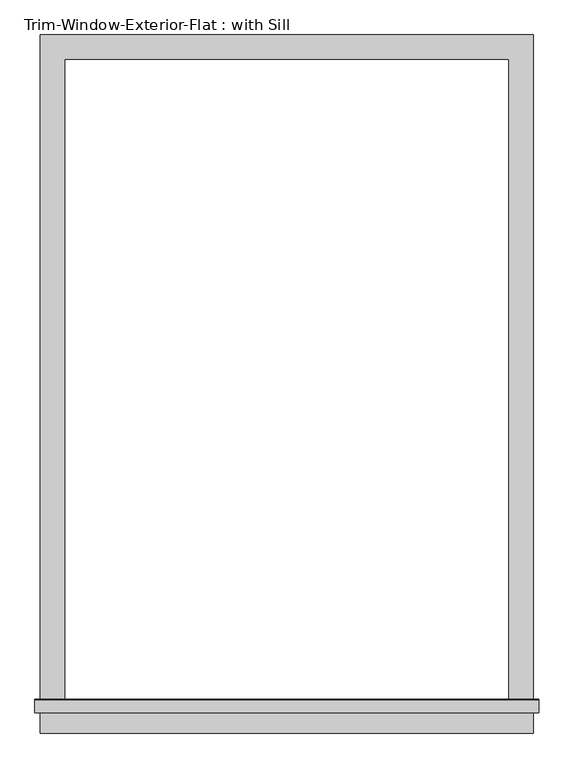
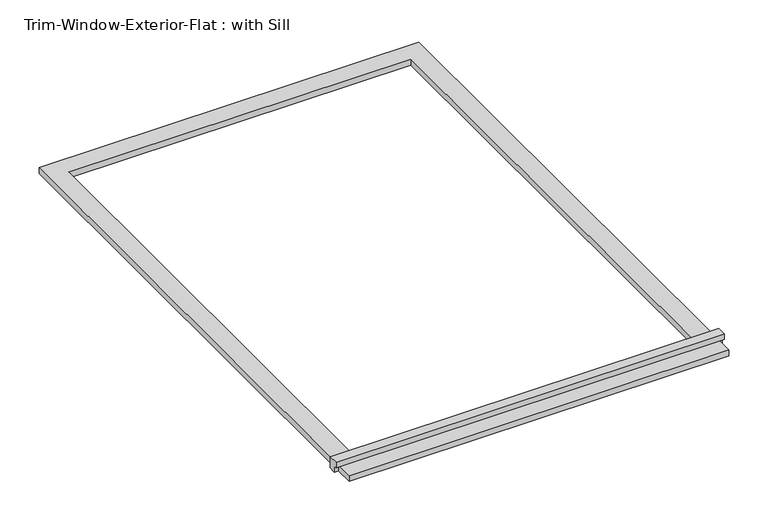
"""IFC4 building model written with IfcOpenShell, lengths in millimetres: proxy geometry, Trim-Window-Exterior-Flat : with Sill."""

import ifcopenshell
import ifcopenshell.guid

model = None  # the IFC model being written
_history = None  # IfcOwnerHistory: only IFC2X3 demands one
_inside = {}  # id of a spatial element -> (the spatial element, [elements in it])
_under = {}  # id of a project, library or spatial element -> (it, [spatial elements below it])
_declared = {}  # id of a project -> (the project, [libraries it declares])
_typed = {}  # id of a type object -> (the type object, [elements of that type])
_made_of = {}  # id of a material, layer set ... -> (it, [elements and type objects made of it])


def new_model(schema):
    """Start an empty IFC model of exactly this schema.

    Asked for "IFC4X3", IfcOpenShell would pick the latest addendum, in which some entities
    have other attributes; the version numbers below select the first issue.
    IFC2X3 requires an IfcOwnerHistory on every rooted entity: one is made here for all.
    """
    global model, _history
    if schema == "IFC4X3":
        model = ifcopenshell.file(schema_version=(4, 3, 0, 0))
    else:
        model = ifcopenshell.file(schema=schema)
    _inside.clear()
    _under.clear()
    _declared.clear()
    _typed.clear()
    _made_of.clear()
    _history = None
    if model.schema == "IFC2X3":
        org = make("IfcOrganization", Name="unknown")
        user = make(
            "IfcPersonAndOrganization",
            ThePerson=make("IfcPerson", FamilyName="unknown"),
            TheOrganization=org,
        )
        app = make(
            "IfcApplication",
            ApplicationDeveloper=org,
            Version="unknown",
            ApplicationFullName="unknown",
            ApplicationIdentifier="unknown",
        )
        _history = make(
            "IfcOwnerHistory",
            OwningUser=user,
            OwningApplication=app,
            ChangeAction="ADDED",
            CreationDate=0,
        )
    return model


def make(cls, **values):
    """One entity of the class cls with the attributes given. An attribute that is None is left unset."""
    return model.create_entity(
        cls, **{name: value for name, value in values.items() if value is not None}
    )


def rooted(cls, **values):
    """An entity with a GlobalId (a new one), such as an element, a storey or a relation."""
    return make(cls, GlobalId=ifcopenshell.guid.new(), OwnerHistory=_history, **values)


def si_unit(unit_type, name, prefix=None):
    """IfcSIUnit, for example si_unit("LENGTHUNIT", "METRE", prefix="MILLI")."""
    return make("IfcSIUnit", UnitType=unit_type, Prefix=prefix, Name=name)


def assignment(units):
    """IfcUnitAssignment: the units of a project."""
    return None if units is None else make("IfcUnitAssignment", Units=units)


def point(xyz):
    """IfcCartesianPoint."""
    return None if xyz is None else make("IfcCartesianPoint", Coordinates=xyz)


def direction(xyz):
    """IfcDirection."""
    return None if xyz is None else make("IfcDirection", DirectionRatios=xyz)


def frame(location, z_axis=None, x_axis=None):
    """IfcAxis2Placement3D, a coordinate frame: its origin and axes. An axis left out is left unset."""
    return make(
        "IfcAxis2Placement3D",
        Location=point(location),
        Axis=direction(z_axis),
        RefDirection=direction(x_axis),
    )


def origin():
    """The frame at (0, 0, 0) with its axes left unset."""
    return frame((0.0, 0.0, 0.0))


def origin_with_axes():
    """The frame at (0, 0, 0) with the z axis (0, 0, 1) and the x axis (1, 0, 0) written out."""
    return frame((0.0, 0.0, 0.0), z_axis=(0.0, 0.0, 1.0), x_axis=(1.0, 0.0, 0.0))


def place(relative_to, where):
    """IfcLocalPlacement: puts the frame where relative to a parent placement (None: the world)."""
    return make(
        "IfcLocalPlacement", PlacementRelTo=relative_to, RelativePlacement=where
    )


def context(
    kind, dimensions, precision=None, world=None, true_north=None, identifier=None
):
    """IfcGeometricRepresentationContext, for example the 3D "Model" context."""
    return make(
        "IfcGeometricRepresentationContext",
        ContextIdentifier=identifier,
        ContextType=kind,
        CoordinateSpaceDimension=dimensions,
        Precision=precision,
        WorldCoordinateSystem=world,
        TrueNorth=true_north,
    )


def project(units=None, contexts=None):
    """IfcProject with its units and contexts."""
    return rooted(
        "IfcProject",
        Name="project",
        RepresentationContexts=contexts,
        UnitsInContext=assignment(units),
    )


def spatial(cls, under=None, at=None, **own):
    """A site, building, storey or space (cls), placed at a placement, below another one or the project."""
    s = rooted(cls, ObjectPlacement=at, **own)
    if under is not None:
        _under.setdefault(under.id(), (under, []))[1].append(s)
    return s


def polyline(points):
    """IfcPolyline through the points."""
    return make("IfcPolyline", Points=[point(p) for p in points])


def outline(outer, holes=None, kind="AREA"):
    """IfcArbitraryClosedProfileDef: a profile drawn as a closed curve; with holes, ...WithVoids."""
    if holes is None:
        return make("IfcArbitraryClosedProfileDef", ProfileType=kind, OuterCurve=outer)
    return make(
        "IfcArbitraryProfileDefWithVoids",
        ProfileType=kind,
        OuterCurve=outer,
        InnerCurves=holes,
    )


def extrude(swept, where, along, depth):
    """IfcExtrudedAreaSolid: the profile swept, set in the frame where, extruded along a direction by depth."""
    return make(
        "IfcExtrudedAreaSolid",
        SweptArea=swept,
        Position=where,
        ExtrudedDirection=direction(along),
        Depth=depth,
    )


def shape(context_of_items, identifier, shape_type, items):
    """IfcShapeRepresentation: the items that make up one representation, for example the "Body"."""
    return make(
        "IfcShapeRepresentation",
        ContextOfItems=context_of_items,
        RepresentationIdentifier=identifier,
        RepresentationType=shape_type,
        Items=items,
    )


def source(mapping_origin, context_of_items, identifier, shape_type, items):
    """IfcRepresentationMap: a shape defined once, which mapped items show again and again."""
    return make(
        "IfcRepresentationMap",
        MappingOrigin=mapping_origin,
        MappedRepresentation=shape(context_of_items, identifier, shape_type, items),
    )


def transform(
    local_origin,
    x_axis=None,
    y_axis=None,
    z_axis=None,
    scale=None,
    scale2=None,
    scale3=None,
    uniform=True,
):
    """IfcCartesianTransformationOperator3D, or its non-uniform kind. x_axis, y_axis, z_axis: its Axis1, 2, 3."""
    if uniform:
        return make(
            "IfcCartesianTransformationOperator3D",
            Axis1=direction(x_axis),
            Axis2=direction(y_axis),
            LocalOrigin=point(local_origin),
            Scale=scale,
            Axis3=direction(z_axis),
        )
    return make(
        "IfcCartesianTransformationOperator3DnonUniform",
        Axis1=direction(x_axis),
        Axis2=direction(y_axis),
        LocalOrigin=point(local_origin),
        Scale=scale,
        Axis3=direction(z_axis),
        Scale2=scale2,
        Scale3=scale3,
    )


def mapped(mapping_source, mapping_target):
    """IfcMappedItem: shows the shape of a source again, moved by a transform."""
    return make(
        "IfcMappedItem", MappingSource=mapping_source, MappingTarget=mapping_target
    )


def made_of(thing, what):
    """Note that an element or type object is made of a material, layer set ...; save() writes the relation."""
    if what is not None:
        _made_of.setdefault(what.id(), (what, []))[1].append(thing)
    return thing


def element(
    cls,
    number,
    at=None,
    inside=None,
    cuts=None,
    type_object=None,
    material=None,
    context=None,
    identifier="Body",
    shape_type=None,
    held_by="IfcProductDefinitionShape",
    body=None,
    shapes=None,
    **own,
):
    """One element of the class cls, such as IfcWall. Its Tag is "e" and its number.

    at: its placement. inside: the storey or other place that contains it. cuts: it is an
    opening in that element (IfcRelVoidsElement). A single representation is given by context,
    identifier, shape_type and body (its items); several are given by shapes. held_by: the class
    of the entity that holds the representations. save() writes the other relations.
    """
    e = rooted(cls, Tag="e%d" % number, ObjectPlacement=at, **own)
    if body is not None:
        shapes = [shape(context, identifier, shape_type, body)]
    if shapes is not None:
        e.Representation = make(held_by, Representations=shapes)
    if inside is not None:
        _inside.setdefault(inside.id(), (inside, []))[1].append(e)
    if cuts is not None:
        rooted(
            "IfcRelVoidsElement", RelatingBuildingElement=cuts, RelatedOpeningElement=e
        )
    if type_object is not None:
        _typed.setdefault(type_object.id(), (type_object, []))[1].append(e)
    return made_of(e, material)


def aggregate(whole, parts):
    """IfcRelAggregates: a whole, such as a stair, and the parts it consists of."""
    return rooted("IfcRelAggregates", RelatingObject=whole, RelatedObjects=parts)


def save(model, path):
    """Write the relations noted so far, then the file.

    IfcRelAggregates (storeys below a building ...), IfcRelContainedInSpatialStructure (elements
    in a storey), IfcRelDefinesByType, IfcRelAssociatesMaterial and IfcRelDeclares: one each for
    every whole, place, type object, material and project.
    """
    for whole, parts in _under.values():
        aggregate(whole, parts)
    for where, things in _inside.values():
        rooted(
            "IfcRelContainedInSpatialStructure",
            RelatedElements=things,
            RelatingStructure=where,
        )
    for kind, things in _typed.values():
        rooted("IfcRelDefinesByType", RelatedObjects=things, RelatingType=kind)
    for what, things in _made_of.values():
        rooted("IfcRelAssociatesMaterial", RelatedObjects=things, RelatingMaterial=what)
    for by, libraries in _declared.values():
        rooted("IfcRelDeclares", RelatingContext=by, RelatedDefinitions=libraries)
    model.write(path)


def trim_window_exterior_flat_with_sill_7e0c1154(model_context):
    return source(origin(), model_context, "Body", "SweptSolid", [
        extrude(outline(polyline([(577.85, -1520.7823709), (577.85, -1577.9323709), (-577.85, -1577.9323709), (-577.85, -1520.7823709), (577.85, -1520.7823709)])), origin_with_axes(), (0.0, 0.0, 1.0), 19.05),
        extrude(outline(polyline([(-1530.35, 38.1), (-1501.0580645, 38.1), (-1498.6, 19.05), (-1498.6, 0.0), (-1520.7823709, 0.0), (-1520.7823709, 19.05), (-1530.35, 19.05), (-1530.35, 38.1)])), frame((-590.55, 0.0, 0.0), z_axis=(1.0, 0.0, 0.0), x_axis=(0.0, 1.0, 0.0)), (0.0, 0.0, 1.0), 1181.1),
        extrude(outline(polyline([(-577.85, 57.15), (577.85, 57.15), (577.85, -1498.6), (520.7, -1498.6), (520.7, 0.0), (-520.7, 0.0), (-520.7, -1498.6), (-577.85, -1498.6), (-577.85, 57.15)])), origin_with_axes(), (0.0, 0.0, 1.0), 19.05),
    ])


if __name__ == "__main__":
    model = new_model("IFC4")
    model_context = context("Model", 3, world=origin())
    ifc_project = project(units=[si_unit("LENGTHUNIT", "METRE", prefix="MILLI")], contexts=[model_context])
    site = spatial("IfcSite", under=ifc_project)
    building = spatial("IfcBuilding", under=site)
    placement = place(None, origin())
    trim_window_exterior_flat_with_sill_shape = trim_window_exterior_flat_with_sill_7e0c1154(model_context)
    element("IfcBuildingElementProxy", 1, Name="Trim-Window-Exterior-Flat : with Sill", ObjectType="Trim-Window-Exterior-Flat : with Sill", at=placement, inside=building, context=model_context, shape_type="MappedRepresentation", body=[
        mapped(trim_window_exterior_flat_with_sill_shape, transform((0.0, 0.0, 0.0), x_axis=(1.0, 0.0, 0.0), y_axis=(0.0, 1.0, 0.0), z_axis=(0.0, 0.0, 1.0))),
    ])
    save(model, "model.ifc")

# Revit data of these elements
# Type "Trim-Window-Exterior-Flat : with Sill"
#   Trim Width = 0' - 2 1/4"
#   Trim Thickness_Picture Frame = 0' - 1 1/4"
#   Trim Thickness_with Sill = 0' - 0 3/4"
#   Sill Thickness = 0' - 1 1/4"
#   Opening Width [instance default] = 2' - 0"
#   Opening Height [instance default] = 3' - 0"
#   Default Elevation = 4' - 0"
#   Sill = yes
#   Picture Frame = no
#   Trim Material [instance default] = none
# Element 1 (IfcBuildingElementProxy, "Trim-Window-Exterior-Flat : with Sill")
#   Opening Width = 3' - 5"
#   Opening Height = 4' - 11"
#   Trim Material = Clad - White
#   Materials on its faces: "Clad - White"
# Materials
#   "Clad - White": class "Wood", colour RGB 242 242 238, transparency 0, Cost = 0
